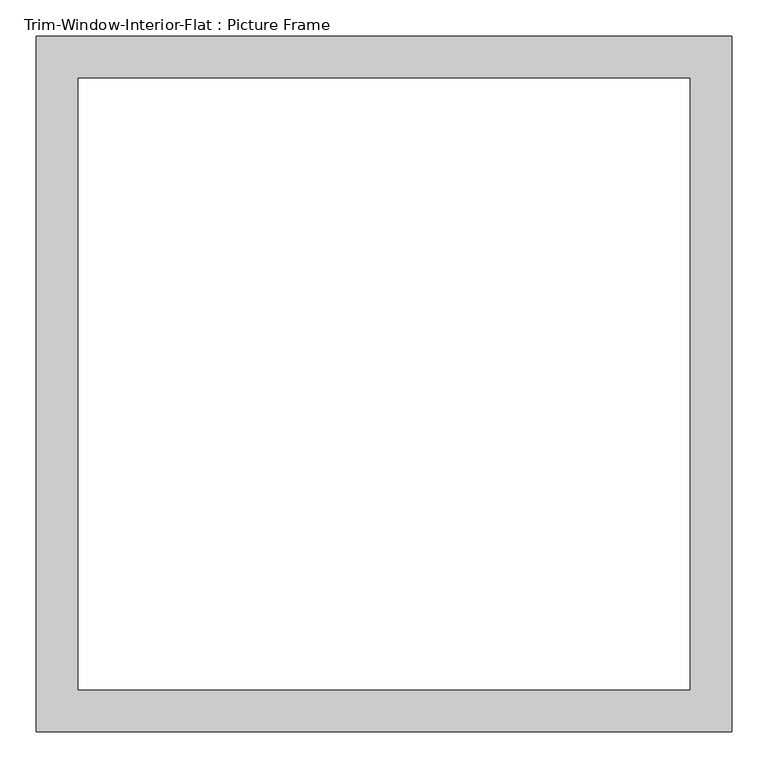
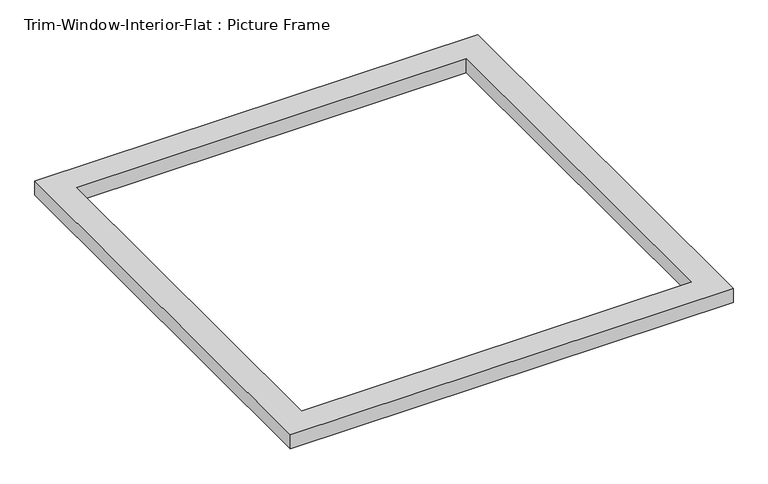
"""IFC4 building model written with IfcOpenShell, lengths in millimetres: proxy geometry, Trim-Window-Interior-Flat : Picture Frame."""

from ifc_helpers import new_model, si_unit, origin, origin_with_axes, place, context, project, spatial, polyline, outline, extrude, source, transform, mapped, element, save


def trim_window_interior_flat_picture_frame_8ff237ef(model_context):
    return source(origin(), model_context, "Body", "SweptSolid", [
        extrude(outline(polyline([(476.25, 44.45), (476.25, -908.05), (-476.25, -908.05), (-476.25, 44.45), (476.25, 44.45)]), holes=[polyline([(419.1, -12.7), (-419.1, -12.7), (-419.1, -850.9), (419.1, -850.9), (419.1, -12.7)])]), origin_with_axes(), (0.0, 0.0, 1.0), 31.75),
    ])


if __name__ == "__main__":
    model = new_model("IFC4")
    model_context = context("Model", 3, world=origin())
    ifc_project = project(units=[si_unit("LENGTHUNIT", "METRE", prefix="MILLI")], contexts=[model_context])
    site = spatial("IfcSite", under=ifc_project)
    building = spatial("IfcBuilding", under=site)
    placement = place(None, origin())
    trim_window_interior_flat_picture_frame_shape = trim_window_interior_flat_picture_frame_8ff237ef(model_context)
    element("IfcBuildingElementProxy", 1, Name="Trim-Window-Interior-Flat : Picture Frame", ObjectType="Trim-Window-Interior-Flat : Picture Frame", at=placement, inside=building, context=model_context, shape_type="MappedRepresentation", body=[
        mapped(trim_window_interior_flat_picture_frame_shape, transform((0.0, 0.0, 0.0), x_axis=(1.0, 0.0, 0.0), y_axis=(0.0, 1.0, 0.0), z_axis=(0.0, 0.0, 1.0))),
    ])
    save(model, "model.ifc")

# Revit data of these elements
# Type "Trim-Window-Interior-Flat : Picture Frame"
#   Trim Thickness_Picture Frame = 0' - 1 1/4"
#   Trim Width = 0' - 2 1/4"
#   Trim Thickness_with Sill = 0' - 0 3/4"
#   Sill Thickness = 0' - 1 1/4"
#   Opening Width [instance default] = 2' - 0"
#   Opening Height [instance default] = 3' - 0"
#   Default Elevation = 4' - 0"
#   Sill = no
#   Picture Frame = yes
#   Trim Material [instance default] = none
# Element 1 (IfcBuildingElementProxy, "Trim-Window-Interior-Flat : Picture Frame")
#   Opening Width = 2' - 10"
#   Opening Height = 2' - 10"
#   Trim Material = 1X WOOD COMPOSITE TRIM
#   Materials on its faces: "1X WOOD COMPOSITE TRIM"
# Materials
#   "1X WOOD COMPOSITE TRIM": class "Generic", colour RGB 88 61 61, transparency 0, Cost = 0
